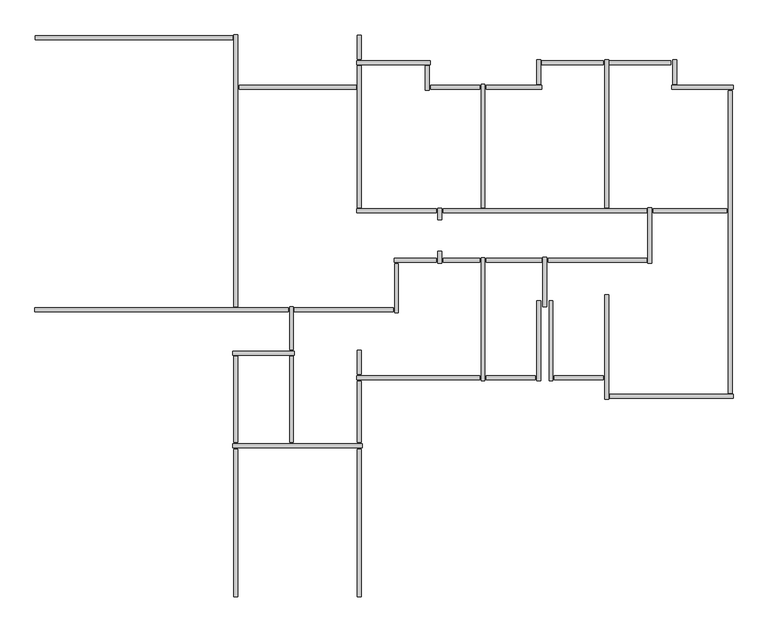
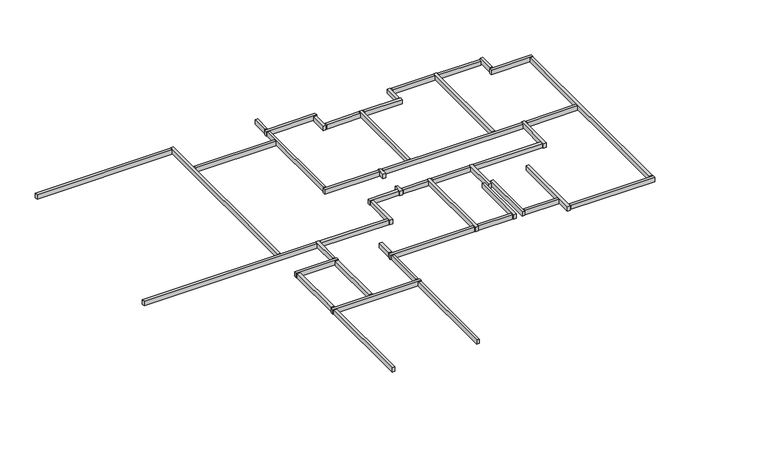
"""IFC4 building model written with IfcOpenShell, lengths in millimetres: beam geometry, Graute viga de respaldo17 : Graute viga de respaldo."""

from ifc_helpers import new_model, si_unit, frame, origin, place, context, project, spatial, polyline, outline, extrude, source, transform, mapped, element, save


def beam_acff9d09(model_context):
    return source(origin(), model_context, "Body", "SweptSolid", [
        extrude(outline(polyline([(-62804.9587292, 72814.9577736), (-62804.9587292, 72720.9577736), (-67594.9587292, 72720.9577736), (-67594.9587292, 72814.9577736), (-62804.9587292, 72814.9577736)])), frame((0.0, 0.0, 14632.9999999), z_axis=(0.0, 0.0, 1.0), x_axis=(1.0, 0.0, 0.0)), (0.0, 0.0, 1.0), 167.0),
        extrude(outline(polyline([(-59771.9587292, 62785.4278788), (-59677.9587292, 62785.4278788), (-59677.9587292, 59195.4278788), (-59771.9587292, 59195.4278788), (-59771.9587292, 62785.4278788)])), frame((0.0, 0.0, 14632.9999999), z_axis=(0.0, 0.0, 1.0), x_axis=(1.0, 0.0, 0.0)), (0.0, 0.0, 1.0), 167.0),
        extrude(outline(polyline([(-62771.9587292, 62785.4278788), (-62677.9587292, 62785.4278788), (-62677.9587292, 59195.4278788), (-62771.9587292, 59195.4278788), (-62771.9587292, 62785.4278788)])), frame((0.0, 0.0, 14632.9999999), z_axis=(0.0, 0.0, 1.0), x_axis=(1.0, 0.0, 0.0)), (0.0, 0.0, 1.0), 167.0),
        extrude(outline(polyline([(-54994.9587292, 64468.4278788), (-54994.9587292, 64562.4278788), (-53804.9587292, 64562.4278788), (-53804.9587292, 64468.4278788), (-54994.9587292, 64468.4278788)])), frame((0.0, 0.0, 14632.9999999), z_axis=(0.0, 0.0, 1.0), x_axis=(1.0, 0.0, 0.0)), (0.0, 0.0, 1.0), 167.0),
        extrude(outline(polyline([(-56644.9587292, 64468.4278788), (-56644.9587292, 64562.4278788), (-55454.9587292, 64562.4278788), (-55454.9587292, 64468.4278788), (-56644.9587292, 64468.4278788)])), frame((0.0, 0.0, 14632.9999999), z_axis=(0.0, 0.0, 1.0), x_axis=(1.0, 0.0, 0.0)), (0.0, 0.0, 1.0), 167.0),
        extrude(outline(polyline([(-52594.9587292, 68518.4278788), (-52594.9587292, 68612.4278788), (-50804.9587292, 68612.4278788), (-50804.9587292, 68518.4278788), (-52594.9587292, 68518.4278788)])), frame((0.0, 0.0, 14632.9999999), z_axis=(0.0, 0.0, 1.0), x_axis=(1.0, 0.0, 0.0)), (0.0, 0.0, 1.0), 167.0),
        extrude(outline(polyline([(-57994.9587292, 71518.4278788), (-57994.9587292, 71612.4278788), (-56804.9587292, 71612.4278788), (-56804.9587292, 71518.4278788), (-57994.9587292, 71518.4278788)])), frame((0.0, 0.0, 14632.9999999), z_axis=(0.0, 0.0, 1.0), x_axis=(1.0, 0.0, 0.0)), (0.0, 0.0, 1.0), 167.0),
        extrude(outline(polyline([(-58027.9587292, 71495.4278788), (-58121.9587292, 71495.4278788), (-58121.9587292, 72085.4278788), (-58027.9587292, 72085.4278788), (-58027.9587292, 71495.4278788)])), frame((0.0, 0.0, 14632.9999999), z_axis=(0.0, 0.0, 1.0), x_axis=(1.0, 0.0, 0.0)), (0.0, 0.0, 1.0), 167.0),
        extrude(outline(polyline([(-59794.9587292, 72118.4278788), (-59794.9587292, 72212.4278788), (-58004.9587292, 72212.4278788), (-58004.9587292, 72118.4278788), (-59794.9587292, 72118.4278788)])), frame((0.0, 0.0, 14632.9999999), z_axis=(0.0, 0.0, 1.0), x_axis=(1.0, 0.0, 0.0)), (0.0, 0.0, 1.0), 167.0),
        extrude(outline(polyline([(-57821.9587292, 68635.4278788), (-57727.9587292, 68635.4278788), (-57727.9587292, 68345.4278788), (-57821.9587292, 68345.4278788), (-57821.9587292, 68635.4278788)])), frame((0.0, 0.0, 14632.9999999), z_axis=(0.0, 0.0, 1.0), x_axis=(1.0, 0.0, 0.0)), (0.0, 0.0, 1.0), 167.0),
        extrude(outline(polyline([(-55144.9587292, 67318.4278788), (-55144.9587292, 67412.4278788), (-52754.9587292, 67412.4278788), (-52754.9587292, 67318.4278788), (-55144.9587292, 67318.4278788)])), frame((0.0, 0.0, 14632.9999999), z_axis=(0.0, 0.0, 1.0), x_axis=(1.0, 0.0, 0.0)), (0.0, 0.0, 1.0), 167.0),
        extrude(outline(polyline([(-56644.9587292, 67318.4278788), (-56644.9587292, 67412.4278788), (-55304.9587292, 67412.4278788), (-55304.9587292, 67318.4278788), (-56644.9587292, 67318.4278788)])), frame((0.0, 0.0, 14632.9999999), z_axis=(0.0, 0.0, 1.0), x_axis=(1.0, 0.0, 0.0)), (0.0, 0.0, 1.0), 167.0),
        extrude(outline(polyline([(-57694.9587292, 67318.4278788), (-57694.9587292, 67412.4278788), (-56804.9587292, 67412.4278788), (-56804.9587292, 67318.4278788), (-57694.9587292, 67318.4278788)])), frame((0.0, 0.0, 14632.9999999), z_axis=(0.0, 0.0, 1.0), x_axis=(1.0, 0.0, 0.0)), (0.0, 0.0, 1.0), 167.0),
        extrude(outline(polyline([(-57821.9587292, 67585.4278788), (-57727.9587292, 67585.4278788), (-57727.9587292, 67295.4278788), (-57821.9587292, 67295.4278788), (-57821.9587292, 67585.4278788)])), frame((0.0, 0.0, 14632.9999999), z_axis=(0.0, 0.0, 1.0), x_axis=(1.0, 0.0, 0.0)), (0.0, 0.0, 1.0), 167.0),
        extrude(outline(polyline([(-58884.9587292, 67318.4278788), (-58884.9587292, 67412.4278788), (-57854.9587292, 67412.4278788), (-57854.9587292, 67318.4278788), (-58884.9587292, 67318.4278788)])), frame((0.0, 0.0, 14632.9999999), z_axis=(0.0, 0.0, 1.0), x_axis=(1.0, 0.0, 0.0)), (0.0, 0.0, 1.0), 167.0),
        extrude(outline(polyline([(-58777.9587292, 66095.4278788), (-58871.9587292, 66095.4278788), (-58871.9587292, 67285.4278788), (-58777.9587292, 67285.4278788), (-58777.9587292, 66095.4278788)])), frame((0.0, 0.0, 14632.9999999), z_axis=(0.0, 0.0, 1.0), x_axis=(1.0, 0.0, 0.0)), (0.0, 0.0, 1.0), 167.0),
        extrude(outline(polyline([(-61304.9587292, 66118.4278788), (-61304.9587292, 66212.4278788), (-58904.9587292, 66212.4278788), (-58904.9587292, 66118.4278788), (-61304.9587292, 66118.4278788)])), frame((0.0, 0.0, 14632.9999999), z_axis=(0.0, 0.0, 1.0), x_axis=(1.0, 0.0, 0.0)), (0.0, 0.0, 1.0), 167.0),
        extrude(outline(polyline([(-56771.9587292, 67430.4278788), (-56677.9587292, 67430.4278788), (-56677.9587292, 64445.4278788), (-56771.9587292, 64445.4278788), (-56771.9587292, 67430.4278788)])), frame((0.0, 0.0, 14632.9999999), z_axis=(0.0, 0.0, 1.0), x_axis=(1.0, 0.0, 0.0)), (0.0, 0.0, 1.0), 167.0),
        extrude(outline(polyline([(-59794.9587292, 64468.4278788), (-59794.9587292, 64562.4278788), (-56804.9587292, 64562.4278788), (-56804.9587292, 64468.4278788), (-59794.9587292, 64468.4278788)])), frame((0.0, 0.0, 14632.9999999), z_axis=(0.0, 0.0, 1.0), x_axis=(1.0, 0.0, 0.0)), (0.0, 0.0, 1.0), 167.0),
        extrude(outline(polyline([(-59771.9587292, 65185.4278788), (-59677.9587292, 65185.4278788), (-59677.9587292, 64595.4278788), (-59771.9587292, 64595.4278788), (-59771.9587292, 65185.4278788)])), frame((0.0, 0.0, 14632.9999999), z_axis=(0.0, 0.0, 1.0), x_axis=(1.0, 0.0, 0.0)), (0.0, 0.0, 1.0), 167.0),
        extrude(outline(polyline([(-59677.9587292, 62945.4278788), (-59771.9587292, 62945.4278788), (-59771.9587292, 64435.4278788), (-59677.9587292, 64435.4278788), (-59677.9587292, 62945.4278788)])), frame((0.0, 0.0, 14632.9999999), z_axis=(0.0, 0.0, 1.0), x_axis=(1.0, 0.0, 0.0)), (0.0, 0.0, 1.0), 167.0),
        extrude(outline(polyline([(-62677.9587292, 62945.4278788), (-62771.9587292, 62945.4278788), (-62771.9587292, 65035.4278788), (-62677.9587292, 65035.4278788), (-62677.9587292, 62945.4278788)])), frame((0.0, 0.0, 14632.9999999), z_axis=(0.0, 0.0, 1.0), x_axis=(1.0, 0.0, 0.0)), (0.0, 0.0, 1.0), 167.0),
        extrude(outline(polyline([(-61327.9587292, 62945.4278788), (-61421.9587292, 62945.4278788), (-61421.9587292, 65035.4278788), (-61327.9587292, 65035.4278788), (-61327.9587292, 62945.4278788)])), frame((0.0, 0.0, 14632.9999999), z_axis=(0.0, 0.0, 1.0), x_axis=(1.0, 0.0, 0.0)), (0.0, 0.0, 1.0), 167.0),
        extrude(outline(polyline([(-61421.9587292, 66235.4278788), (-61327.9587292, 66235.4278788), (-61327.9587292, 65195.4278788), (-61421.9587292, 65195.4278788), (-61421.9587292, 66235.4278788)])), frame((0.0, 0.0, 14632.9999999), z_axis=(0.0, 0.0, 1.0), x_axis=(1.0, 0.0, 0.0)), (0.0, 0.0, 1.0), 167.0),
        extrude(outline(polyline([(-62644.9587292, 71518.4278788), (-62644.9587292, 71612.4278788), (-59804.9587292, 71612.4278788), (-59804.9587292, 71518.4278788), (-62644.9587292, 71518.4278788)])), frame((0.0, 0.0, 14632.9999999), z_axis=(0.0, 0.0, 1.0), x_axis=(1.0, 0.0, 0.0)), (0.0, 0.0, 1.0), 167.0),
        extrude(outline(polyline([(-59677.9587292, 68645.4278788), (-59771.9587292, 68645.4278788), (-59771.9587292, 72085.4278788), (-59677.9587292, 72085.4278788), (-59677.9587292, 68645.4278788)])), frame((0.0, 0.0, 14632.9999999), z_axis=(0.0, 0.0, 1.0), x_axis=(1.0, 0.0, 0.0)), (0.0, 0.0, 1.0), 167.0),
        extrude(outline(polyline([(-59794.9587292, 68518.4278788), (-59794.9587292, 68612.4278788), (-57854.9587292, 68612.4278788), (-57854.9587292, 68518.4278788), (-59794.9587292, 68518.4278788)])), frame((0.0, 0.0, 14632.9999999), z_axis=(0.0, 0.0, 1.0), x_axis=(1.0, 0.0, 0.0)), (0.0, 0.0, 1.0), 167.0),
        extrude(outline(polyline([(-57694.9587292, 68518.4278788), (-57694.9587292, 68612.4278788), (-52754.9587292, 68612.4278788), (-52754.9587292, 68518.4278788), (-57694.9587292, 68518.4278788)])), frame((0.0, 0.0, 14632.9999999), z_axis=(0.0, 0.0, 1.0), x_axis=(1.0, 0.0, 0.0)), (0.0, 0.0, 1.0), 167.0),
        extrude(outline(polyline([(-56771.9587292, 71635.4278788), (-56677.9587292, 71635.4278788), (-56677.9587292, 68645.4278788), (-56771.9587292, 68645.4278788), (-56771.9587292, 71635.4278788)])), frame((0.0, 0.0, 14632.9999999), z_axis=(0.0, 0.0, 1.0), x_axis=(1.0, 0.0, 0.0)), (0.0, 0.0, 1.0), 167.0),
        extrude(outline(polyline([(-55304.9587292, 71612.4278788), (-55304.9587292, 71518.4278788), (-56644.9587292, 71518.4278788), (-56644.9587292, 71612.4278788), (-55304.9587292, 71612.4278788)])), frame((0.0, 0.0, 14632.9999999), z_axis=(0.0, 0.0, 1.0), x_axis=(1.0, 0.0, 0.0)), (0.0, 0.0, 1.0), 167.0),
        extrude(outline(polyline([(-55421.9587292, 72235.4278788), (-55327.9587292, 72235.4278788), (-55327.9587292, 71645.4278788), (-55421.9587292, 71645.4278788), (-55421.9587292, 72235.4278788)])), frame((0.0, 0.0, 14632.9999999), z_axis=(0.0, 0.0, 1.0), x_axis=(1.0, 0.0, 0.0)), (0.0, 0.0, 1.0), 167.0),
        extrude(outline(polyline([(-55294.9587292, 72118.4278788), (-55294.9587292, 72212.4278788), (-53804.9587292, 72212.4278788), (-53804.9587292, 72118.4278788), (-55294.9587292, 72118.4278788)])), frame((0.0, 0.0, 14632.9999999), z_axis=(0.0, 0.0, 1.0), x_axis=(1.0, 0.0, 0.0)), (0.0, 0.0, 1.0), 167.0),
        extrude(outline(polyline([(-52165.9809043, 72212.4278788), (-52165.9809043, 72117.4278788), (-53654.9587292, 72117.4278788), (-53654.9587292, 72212.4278788), (-52165.9809043, 72212.4278788)])), frame((0.0, 0.0, 14617.1856208), z_axis=(0.0, 0.0, 1.0), x_axis=(1.0, 0.0, 0.0)), (0.0, 0.0, 1.0), 165.0),
        extrude(outline(polyline([(-50677.9587292, 64145.4278788), (-50771.9587292, 64145.4278788), (-50771.9587292, 71485.4278788), (-50677.9587292, 71485.4278788), (-50677.9587292, 64145.4278788)])), frame((0.0, 0.0, 14632.9999999), z_axis=(0.0, 0.0, 1.0), x_axis=(1.0, 0.0, 0.0)), (0.0, 0.0, 1.0), 167.0),
        extrude(outline(polyline([(-52627.9587292, 67295.4278788), (-52721.9587292, 67295.4278788), (-52721.9587292, 68640.7810915), (-52627.9587292, 68640.7810915), (-52627.9587292, 67295.4278788)])), frame((0.0, 0.0, 14632.9999999), z_axis=(0.0, 0.0, 1.0), x_axis=(1.0, 0.0, 0.0)), (0.0, 0.0, 1.0), 167.0),
        extrude(outline(polyline([(-55177.9587292, 66245.4278788), (-55271.9587292, 66245.4278788), (-55271.9587292, 67435.4278788), (-55177.9587292, 67435.4278788), (-55177.9587292, 66245.4278788)])), frame((0.0, 0.0, 14632.9999999), z_axis=(0.0, 0.0, 1.0), x_axis=(1.0, 0.0, 0.0)), (0.0, 0.0, 1.0), 167.0),
        extrude(outline(polyline([(-55027.9587292, 64445.4278788), (-55121.9587292, 64445.4278788), (-55121.9587292, 66385.4278788), (-55027.9587292, 66385.4278788), (-55027.9587292, 64445.4278788)])), frame((0.0, 0.0, 14632.9999999), z_axis=(0.0, 0.0, 1.0), x_axis=(1.0, 0.0, 0.0)), (0.0, 0.0, 1.0), 167.0),
        extrude(outline(polyline([(-55327.9587292, 64445.4278788), (-55421.9587292, 64445.4278788), (-55421.9587292, 66385.4278788), (-55327.9587292, 66385.4278788), (-55327.9587292, 64445.4278788)])), frame((0.0, 0.0, 14632.9999999), z_axis=(0.0, 0.0, 1.0), x_axis=(1.0, 0.0, 0.0)), (0.0, 0.0, 1.0), 167.0),
        extrude(outline(polyline([(-53677.9587292, 63995.4278788), (-53771.9587292, 63995.4278788), (-53771.9587292, 66535.4278788), (-53677.9587292, 66535.4278788), (-53677.9587292, 63995.4278788)])), frame((0.0, 0.0, 14632.9999999), z_axis=(0.0, 0.0, 1.0), x_axis=(1.0, 0.0, 0.0)), (0.0, 0.0, 1.0), 167.0),
        extrude(outline(polyline([(-50654.9587292, 64112.4278788), (-50654.9587292, 64018.4278788), (-53644.9587292, 64018.4278788), (-53644.9587292, 64112.4278788), (-50654.9587292, 64112.4278788)])), frame((0.0, 0.0, 14632.9999999), z_axis=(0.0, 0.0, 1.0), x_axis=(1.0, 0.0, 0.0)), (0.0, 0.0, 1.0), 167.0),
        extrude(outline(polyline([(-52121.9587292, 72235.4278788), (-52027.9587292, 72235.4278788), (-52027.9587292, 71645.4278788), (-52121.9587292, 71645.4278788), (-52121.9587292, 72235.4278788)])), frame((0.0, 0.0, 14632.9999999), z_axis=(0.0, 0.0, 1.0), x_axis=(1.0, 0.0, 0.0)), (0.0, 0.0, 1.0), 167.0),
        extrude(outline(polyline([(-52144.9587292, 71518.4278788), (-52144.9587292, 71612.4278788), (-50654.9587292, 71612.4278788), (-50654.9587292, 71518.4278788), (-52144.9587292, 71518.4278788)])), frame((0.0, 0.0, 14632.9999999), z_axis=(0.0, 0.0, 1.0), x_axis=(1.0, 0.0, 0.0)), (0.0, 0.0, 1.0), 167.0),
        extrude(outline(polyline([(-53771.9587292, 72235.4278788), (-53677.9587292, 72235.4278788), (-53677.9587292, 68645.4278788), (-53771.9587292, 68645.4278788), (-53771.9587292, 72235.4278788)])), frame((0.0, 0.0, 14632.9999999), z_axis=(0.0, 0.0, 1.0), x_axis=(1.0, 0.0, 0.0)), (0.0, 0.0, 1.0), 167.0),
        extrude(outline(polyline([(-59771.9587292, 72835.4278788), (-59677.9587292, 72835.4278788), (-59677.9587292, 72245.4278788), (-59771.9587292, 72245.4278788), (-59771.9587292, 72835.4278788)])), frame((0.0, 0.0, 14632.9999999), z_axis=(0.0, 0.0, 1.0), x_axis=(1.0, 0.0, 0.0)), (0.0, 0.0, 1.0), 167.0),
        extrude(outline(polyline([(-62794.9587292, 65068.4278788), (-62794.9587292, 65162.4278788), (-61304.9587292, 65162.4278788), (-61304.9587292, 65068.4278788), (-62794.9587292, 65068.4278788)])), frame((0.0, 0.0, 14632.9999999), z_axis=(0.0, 0.0, 1.0), x_axis=(1.0, 0.0, 0.0)), (0.0, 0.0, 1.0), 167.0),
        extrude(outline(polyline([(-62794.9587292, 62818.4278788), (-62794.9587292, 62912.4278788), (-59654.9587292, 62912.4278788), (-59654.9587292, 62818.4278788), (-62794.9587292, 62818.4278788)])), frame((0.0, 0.0, 14632.9999999), z_axis=(0.0, 0.0, 1.0), x_axis=(1.0, 0.0, 0.0)), (0.0, 0.0, 1.0), 167.0),
        extrude(outline(polyline([(-67601.7587292, 66118.4278788), (-67601.7587292, 66212.4278788), (-61454.9587292, 66212.4278788), (-61454.9587292, 66118.4278788), (-67601.7587292, 66118.4278788)])), frame((0.0, 0.0, 14632.9999999), z_axis=(0.0, 0.0, 1.0), x_axis=(1.0, 0.0, 0.0)), (0.0, 0.0, 1.0), 167.0),
        extrude(outline(polyline([(-62771.9587292, 72837.9577736), (-62677.9587292, 72837.9577736), (-62677.9587292, 66245.4278788), (-62771.9587292, 66245.4278788), (-62771.9587292, 72837.9577736)])), frame((0.0, 0.0, 14632.9999999), z_axis=(0.0, 0.0, 1.0), x_axis=(1.0, 0.0, 0.0)), (0.0, 0.0, 1.0), 167.0),
    ])


if __name__ == "__main__":
    model = new_model("IFC4")
    model_context = context("Model", 3, world=origin())
    ifc_project = project(units=[si_unit("LENGTHUNIT", "METRE", prefix="MILLI")], contexts=[model_context])
    site = spatial("IfcSite", under=ifc_project)
    building = spatial("IfcBuilding", under=site)
    placement = place(None, origin())
    beam_shape = beam_acff9d09(model_context)
    element("IfcBeam", 1, ObjectType="Graute viga de respaldo17 : Graute viga de respaldo", at=placement, inside=building, context=model_context, shape_type="MappedRepresentation", body=[
        mapped(beam_shape, transform((0.0, 0.0, 0.0), x_axis=(1.0, 0.0, 0.0), y_axis=(0.0, 1.0, 0.0), z_axis=(0.0, 0.0, 1.0))),
    ])
    save(model, "model.ifc")

# Revit data of these elements
# Element 1 (IfcBeam, "Graute viga de respaldo17 : Graute viga de respaldo")
#   Materials on its faces: "Concreto, Faixa de areia/cimento"
# Materials
#   "Concreto, Faixa de areia/cimento": class "Concreto", colour RGB 127 127 127, transparency 0, Description = "Revestimento de laje de concreto", Cost = 0
